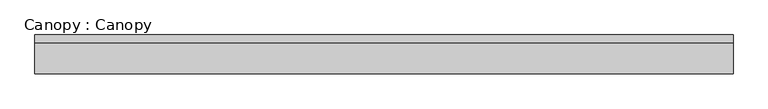
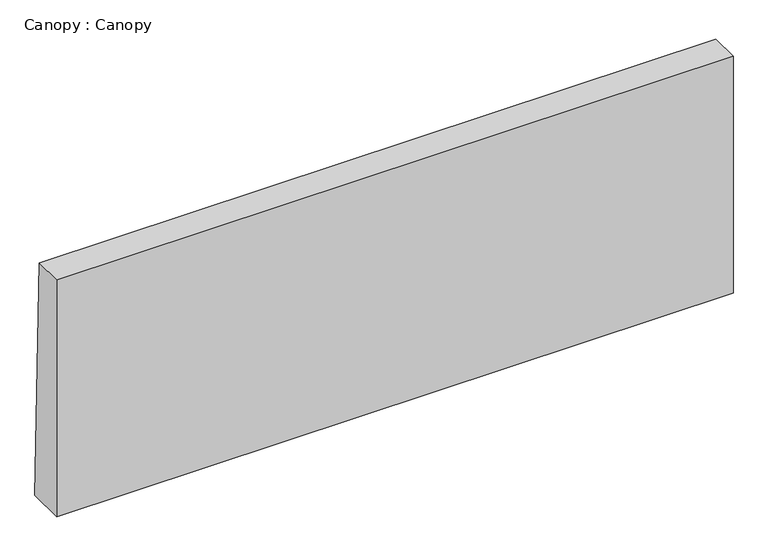
"""IFC4 building model written with IfcOpenShell, lengths in millimetres: proxy geometry, Canopy : Canopy."""

from ifc_helpers import new_model, si_unit, frame, origin, place, context, project, spatial, polyline, outline, extrude, source, transform, mapped, element, save


def canopy_canopy_1427068a(model_context):
    return source(origin(), model_context, "Body", "SweptSolid", [
        extrude(outline(polyline([(150.0, 0.0), (0.0, 0.0), (0.0, 1000.0), (120.0, 1000.0), (150.0, 0.0)])), frame((-1350.0, 0.0, 0.0), z_axis=(1.0, 0.0, 0.0), x_axis=(0.0, 1.0, 0.0)), (0.0, 0.0, 1.0), 2700.0),
    ])


if __name__ == "__main__":
    model = new_model("IFC4")
    model_context = context("Model", 3, world=origin())
    ifc_project = project(units=[si_unit("LENGTHUNIT", "METRE", prefix="MILLI")], contexts=[model_context])
    site = spatial("IfcSite", under=ifc_project)
    building = spatial("IfcBuilding", under=site)
    placement = place(None, origin())
    canopy_canopy_shape = canopy_canopy_1427068a(model_context)
    element("IfcBuildingElementProxy", 1, Name="Canopy : Canopy", ObjectType="Canopy : Canopy", at=placement, inside=building, context=model_context, shape_type="MappedRepresentation", body=[
        mapped(canopy_canopy_shape, transform((0.0, 0.0, 0.0), x_axis=(1.0, 0.0, 0.0), y_axis=(0.0, 1.0, 0.0), z_axis=(0.0, 0.0, 1.0))),
    ])
    save(model, "model.ifc")

# Revit data of these elements
# Type "Canopy : Canopy"
#   Type Comments = "CV-AG"
#   H_Rebar Ratio = 0.1
#   Canopy Width [instance default] = 1700 mm
#   Canopy Length [instance default] = 1000 mm
#   Canopy L.P = 120 mm
#   Canopy H.P = 150 mm
#   구조재료 = Concrete_f'c=28MPa(Cylender)
#   Default Elevation = 0
# Element 1 (IfcBuildingElementProxy, "Canopy : Canopy")
#   Canopy Width = 2700 mm
#   Materials on its faces: "Concrete_f'c=28MPa(Cylender)"
# Materials
#   "Concrete_f'c=28MPa(Cylender)": class "Concrete", colour RGB 176 176 176, transparency 0, Description = "Reinf. Conc.", Cost = 0, Image = Concrete.Cast-In-Place.Flat.Polished.Grey.jpg
